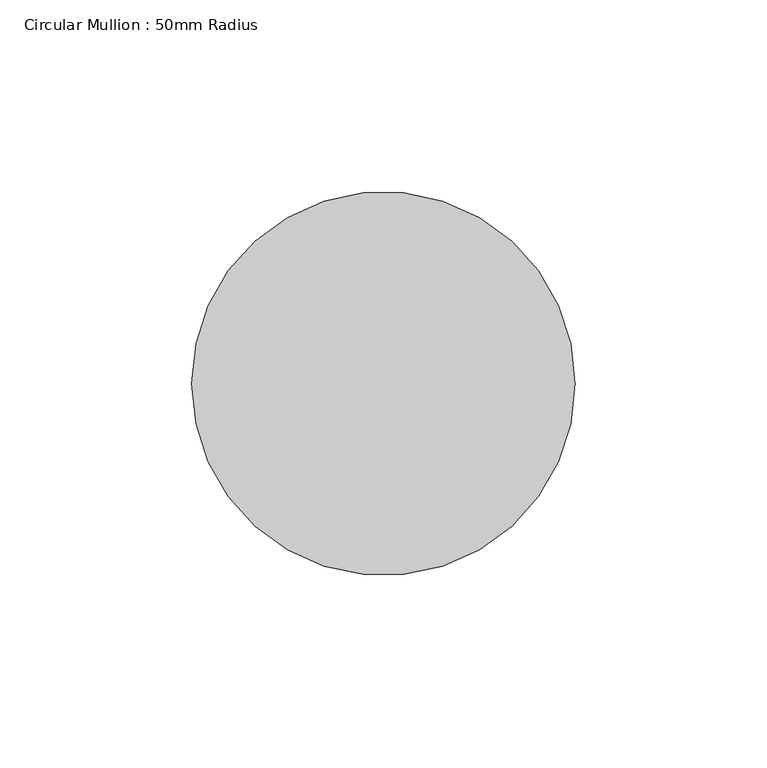
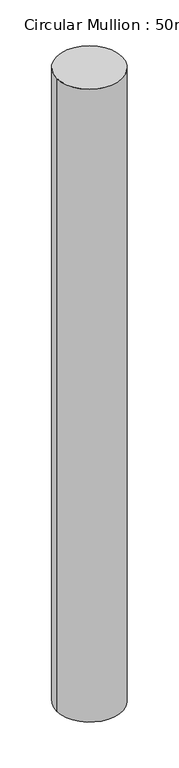
"""IFC4 building model written with IfcOpenShell, lengths in millimetres: member geometry, Circular Mullion : 50mm Radius."""

from ifc_helpers import new_model, si_unit, point, frame, origin, origin_2d, place, context, project, spatial, circle_curve, trimmed, segment, composite_curve, outline, extrude, source, transform, mapped, element, save


def circular_mullion_50mm_radius_0ee57fcc(model_context):
    return source(origin(), model_context, "Body", "SweptSolid", [
        extrude(outline(composite_curve([segment(trimmed(circle_curve(origin_2d(), 50.0), [point((50.0, 0.0))], [point((-50.0, 0.0))], False, "CARTESIAN"), True, "CONTINUOUS"), segment(trimmed(circle_curve(origin_2d(), 50.0), [point((-50.0, 0.0))], [point((50.0, 0.0))], False, "CARTESIAN"), True, "CONTINUOUS")], self_intersect=False)), frame((0.0, 0.0, -1019.5607638), z_axis=(0.0, 0.0, 1.0), x_axis=(1.0, 0.0, 0.0)), (0.0, 0.0, 1.0), 1019.5607638),
    ])


if __name__ == "__main__":
    model = new_model("IFC4")
    model_context = context("Model", 3, world=origin())
    ifc_project = project(units=[si_unit("LENGTHUNIT", "METRE", prefix="MILLI")], contexts=[model_context])
    site = spatial("IfcSite", under=ifc_project)
    building = spatial("IfcBuilding", under=site)
    placement = place(None, origin())
    circular_mullion_50mm_radius_shape = circular_mullion_50mm_radius_0ee57fcc(model_context)
    element("IfcMember", 1, ObjectType="Circular Mullion : 50mm Radius", at=placement, inside=building, context=model_context, shape_type="MappedRepresentation", body=[
        mapped(circular_mullion_50mm_radius_shape, transform((0.0, 0.0, 0.0), x_axis=(1.0, 0.0, 0.0), y_axis=(0.0, 1.0, 0.0), z_axis=(0.0, 0.0, 1.0))),
    ])
    save(model, "model.ifc")

# Revit data of these elements
# Type "Circular Mullion : 50mm Radius"
#   built-in parameter 1007350 = 0.164042 (stored number, unit not read)
# Element 1 (IfcMember, "Circular Mullion : 50mm Radius")
#   Materials on its faces: "Aluminium"
# Materials
#   "Aluminium": class "Metal", colour RGB 247 247 247, transparency 0, Description = "Aluminium 6061", Cost = 0
